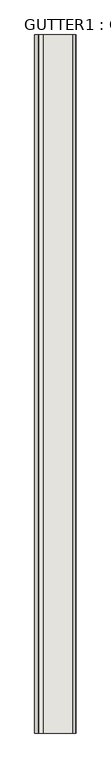
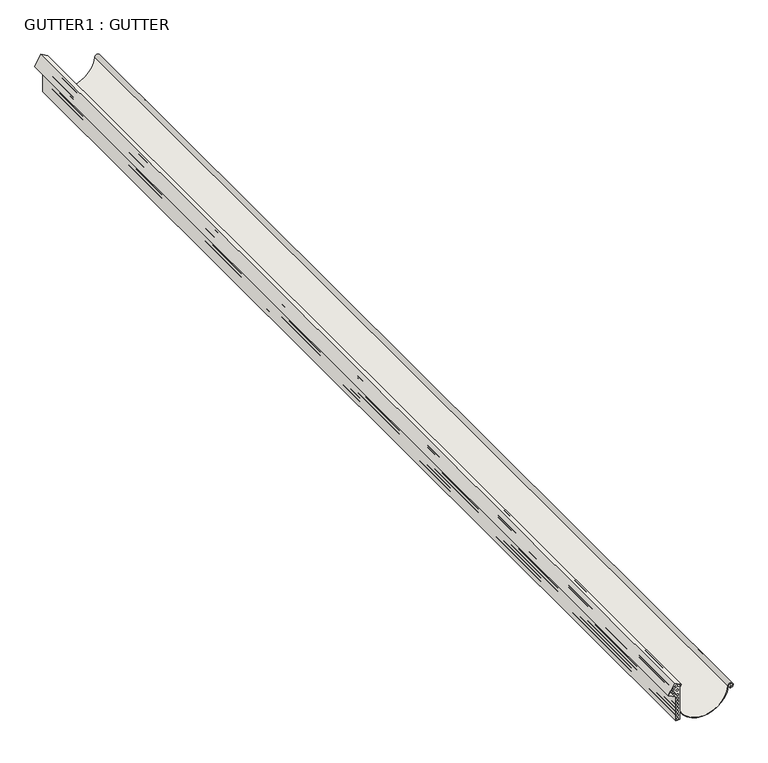
"""IFC4 building model written with IfcOpenShell, lengths in millimetres: wall geometry, GUTTER1 : GUTTER."""

from ifc_helpers import new_model, si_unit, point, frame, frame_2d, origin, place, context, project, spatial, polyline, circle_curve, trimmed, segment, composite_curve, outline, extrude, source, transform, mapped, element, save


def gutter1_gutter_43049d00(model_context):
    return source(origin(), model_context, "Body", "SweptSolid", [
        extrude(outline(composite_curve([segment(polyline([(4096.5843057, 23878.4225998), (4160.0634175, 23878.4225998), (4168.1357989, 23882.3597633), (4178.0149745, 23863.7797363), (4148.9430413, 23848.3219152), (4138.9178689, 23868.8765647), (4072.6574319, 23868.8765647), (4072.6574319, 23878.4225998), (4094.6010309, 23878.4225998)]), True, "CONTINUOUS"), segment(trimmed(circle_curve(frame_2d((4128.5015564, 23937.7583414)), 68.3372216), [point((4094.6010309, 23878.4225998))], [point((4119.7111617, 24005.5278392))], False, "CARTESIAN"), True, "CONTINUOUS"), segment(trimmed(circle_curve(frame_2d((4120.3368331, 24011.223521)), 5.7299439), [point((4119.7111617, 24005.5278392))], [point((4114.6622825, 24010.4287049))], True, "CARTESIAN"), True, "CONTINUOUS"), segment(polyline([(4114.6622825, 24010.4287049), (4119.5801459, 24012.1220611), (4119.8932927, 24011.212617), (4113.9672347, 24009.1721116)]), True, "CONTINUOUS"), segment(trimmed(circle_curve(frame_2d((4120.3368331, 24011.223521)), 6.6917907), [point((4113.9672347, 24009.1721116))], [point((4119.7255439, 24004.5597092))], False, "CARTESIAN"), True, "CONTINUOUS"), segment(trimmed(circle_curve(frame_2d((4128.5015564, 23937.7583414)), 67.3753748), [point((4119.7255439, 24004.5597092))], [point((4096.5843057, 23878.4225998))], True, "CARTESIAN"), True, "CONTINUOUS")], self_intersect=False), holes=[composite_curve([segment(trimmed(circle_curve(frame_2d((4076.5699194, 23873.0369591)), 2.3644757), [point((4076.5699194, 23870.6724834))], [point((4076.5699194, 23875.4014348))], True, "CARTESIAN"), True, "CONTINUOUS"), segment(trimmed(circle_curve(frame_2d((4076.5699194, 23873.0369591)), 2.3644757), [point((4076.5699194, 23875.4014348))], [point((4076.5699194, 23870.6724834))], True, "CARTESIAN"), True, "CONTINUOUS")], self_intersect=False), composite_curve([segment(trimmed(circle_curve(frame_2d((4086.0949194, 23873.0369591)), 2.3644757), [point((4086.0949194, 23870.6724834))], [point((4086.0949194, 23875.4014348))], True, "CARTESIAN"), True, "CONTINUOUS"), segment(trimmed(circle_curve(frame_2d((4086.0949194, 23873.0369591)), 2.3644757), [point((4086.0949194, 23875.4014348))], [point((4086.0949194, 23870.6724834))], True, "CARTESIAN"), True, "CONTINUOUS")], self_intersect=False), composite_curve([segment(trimmed(circle_curve(frame_2d((4095.6199194, 23873.0369591)), 2.3644757), [point((4095.6199194, 23870.6724834))], [point((4095.6199194, 23875.4014348))], True, "CARTESIAN"), True, "CONTINUOUS"), segment(trimmed(circle_curve(frame_2d((4095.6199194, 23873.0369591)), 2.3644757), [point((4095.6199194, 23875.4014348))], [point((4095.6199194, 23870.6724834))], True, "CARTESIAN"), True, "CONTINUOUS")], self_intersect=False), composite_curve([segment(trimmed(circle_curve(frame_2d((4105.1449194, 23873.0369591)), 2.3644757), [point((4105.1449194, 23870.6724834))], [point((4105.1449194, 23875.4014348))], True, "CARTESIAN"), True, "CONTINUOUS"), segment(trimmed(circle_curve(frame_2d((4105.1449194, 23873.0369591)), 2.3644757), [point((4105.1449194, 23875.4014348))], [point((4105.1449194, 23870.6724834))], True, "CARTESIAN"), True, "CONTINUOUS")], self_intersect=False), composite_curve([segment(trimmed(circle_curve(frame_2d((4114.6699194, 23873.0369591)), 2.3644757), [point((4114.6699194, 23870.6724834))], [point((4114.6699194, 23875.4014348))], True, "CARTESIAN"), True, "CONTINUOUS"), segment(trimmed(circle_curve(frame_2d((4114.6699194, 23873.0369591)), 2.3644757), [point((4114.6699194, 23875.4014348))], [point((4114.6699194, 23870.6724834))], True, "CARTESIAN"), True, "CONTINUOUS")], self_intersect=False), composite_curve([segment(trimmed(circle_curve(frame_2d((4124.1949194, 23873.0369591)), 2.3644757), [point((4124.1949194, 23870.6724834))], [point((4124.1949194, 23875.4014348))], True, "CARTESIAN"), True, "CONTINUOUS"), segment(trimmed(circle_curve(frame_2d((4124.1949194, 23873.0369591)), 2.3644757), [point((4124.1949194, 23875.4014348))], [point((4124.1949194, 23870.6724834))], True, "CARTESIAN"), True, "CONTINUOUS")], self_intersect=False), composite_curve([segment(trimmed(circle_curve(frame_2d((4133.7199194, 23873.0369591)), 2.3644757), [point((4133.7199194, 23870.6724834))], [point((4133.7199194, 23875.4014348))], True, "CARTESIAN"), True, "CONTINUOUS"), segment(trimmed(circle_curve(frame_2d((4133.7199194, 23873.0369591)), 2.3644757), [point((4133.7199194, 23875.4014348))], [point((4133.7199194, 23870.6724834))], True, "CARTESIAN"), True, "CONTINUOUS")], self_intersect=False), composite_curve([segment(trimmed(circle_curve(frame_2d((4143.2449194, 23873.0369591)), 2.3644757), [point((4143.2449194, 23870.6724834))], [point((4143.2449194, 23875.4014348))], True, "CARTESIAN"), True, "CONTINUOUS"), segment(trimmed(circle_curve(frame_2d((4143.2449194, 23873.0369591)), 2.3644757), [point((4143.2449194, 23875.4014348))], [point((4143.2449194, 23870.6724834))], True, "CARTESIAN"), True, "CONTINUOUS")], self_intersect=False), composite_curve([segment(trimmed(circle_curve(frame_2d((4167.2721617, 23876.1808019)), 2.3644757), [point((4167.2721617, 23873.8163262))], [point((4167.2721617, 23878.5452775))], True, "CARTESIAN"), True, "CONTINUOUS"), segment(trimmed(circle_curve(frame_2d((4167.2721617, 23876.1808019)), 2.3644757), [point((4167.2721617, 23878.5452775))], [point((4167.2721617, 23873.8163262))], True, "CARTESIAN"), True, "CONTINUOUS")], self_intersect=False), composite_curve([segment(trimmed(circle_curve(frame_2d((4156.0538228, 23872.0976604)), 2.3644757), [point((4156.0538228, 23869.7331848))], [point((4156.0538228, 23874.4621361))], True, "CARTESIAN"), True, "CONTINUOUS"), segment(trimmed(circle_curve(frame_2d((4156.0538228, 23872.0976604)), 2.3644757), [point((4156.0538228, 23874.4621361))], [point((4156.0538228, 23869.7331848))], True, "CARTESIAN"), True, "CONTINUOUS")], self_intersect=False), composite_curve([segment(trimmed(circle_curve(frame_2d((4167.7312491, 23869.6155469)), 2.3644757), [point((4166.4782678, 23867.6103578))], [point((4168.9842303, 23871.6207359))], True, "CARTESIAN"), True, "CONTINUOUS"), segment(trimmed(circle_curve(frame_2d((4167.7312491, 23869.6155469)), 2.3644757), [point((4168.9842303, 23871.6207359))], [point((4166.4782678, 23867.6103578))], True, "CARTESIAN"), True, "CONTINUOUS")], self_intersect=False), composite_curve([segment(trimmed(circle_curve(frame_2d((4164.6415221, 23863.8046156)), 2.3644757), [point((4162.5163455, 23862.7680977))], [point((4166.7666988, 23864.8411335))], True, "CARTESIAN"), True, "CONTINUOUS"), segment(trimmed(circle_curve(frame_2d((4164.6415221, 23863.8046156)), 2.3644757), [point((4166.7666988, 23864.8411335))], [point((4162.5163455, 23862.7680977))], True, "CARTESIAN"), True, "CONTINUOUS")], self_intersect=False), composite_curve([segment(trimmed(circle_curve(frame_2d((4158.9419607, 23860.5139723)), 2.3644757), [point((4156.5904378, 23860.7611273))], [point((4161.2934835, 23860.2668173))], True, "CARTESIAN"), True, "CONTINUOUS"), segment(trimmed(circle_curve(frame_2d((4158.9419607, 23860.5139723)), 2.3644757), [point((4161.2934835, 23860.2668173))], [point((4156.5904378, 23860.7611273))], True, "CARTESIAN"), True, "CONTINUOUS")], self_intersect=False), composite_curve([segment(trimmed(circle_curve(frame_2d((4152.3646831, 23860.7436559)), 2.3644757), [point((4150.5014509, 23862.1993724))], [point((4154.2279154, 23859.2879393))], True, "CARTESIAN"), True, "CONTINUOUS"), segment(trimmed(circle_curve(frame_2d((4152.3646831, 23860.7436559)), 2.3644757), [point((4154.2279154, 23859.2879393))], [point((4150.5014509, 23862.1993724))], True, "CARTESIAN"), True, "CONTINUOUS")], self_intersect=False), composite_curve([segment(trimmed(circle_curve(frame_2d((4146.9085492, 23864.4238647)), 2.3644757), [point((4146.0998509, 23866.645745))], [point((4147.7172475, 23862.2019843))], True, "CARTESIAN"), True, "CONTINUOUS"), segment(trimmed(circle_curve(frame_2d((4146.9085492, 23864.4238647)), 2.3644757), [point((4147.7172475, 23862.2019843))], [point((4146.0998509, 23866.645745))], True, "CARTESIAN"), True, "CONTINUOUS")], self_intersect=False)]), frame((0.0, -3415.0384634, 0.0), z_axis=(0.0, 1.0, 0.0), x_axis=(0.0, 0.0, 1.0)), (0.0, 0.0, 1.0), 2862.7206389),
    ])


if __name__ == "__main__":
    model = new_model("IFC4")
    model_context = context("Model", 3, world=origin())
    ifc_project = project(units=[si_unit("LENGTHUNIT", "METRE", prefix="MILLI")], contexts=[model_context])
    site = spatial("IfcSite", under=ifc_project)
    building = spatial("IfcBuilding", under=site)
    placement = place(None, origin())
    gutter1_gutter_shape = gutter1_gutter_43049d00(model_context)
    element("IfcWall", 1, ObjectType="GUTTER1 : GUTTER", at=placement, inside=building, context=model_context, shape_type="MappedRepresentation", body=[
        mapped(gutter1_gutter_shape, transform((0.0, 0.0, 0.0), x_axis=(1.0, 0.0, 0.0), y_axis=(0.0, 1.0, 0.0), z_axis=(0.0, 0.0, 1.0))),
    ])
    save(model, "model.ifc")

# Revit data of these elements
# Element 1 (IfcWall, "GUTTER1 : GUTTER")
#   Materials on its faces: "HALF ROUND GUTTER - 5\""
# Materials
#   "HALF ROUND GUTTER - 5\"": class "Metal", colour RGB 247 247 247, transparency 0, Description = "Aluminum 6061", Cost = 0
